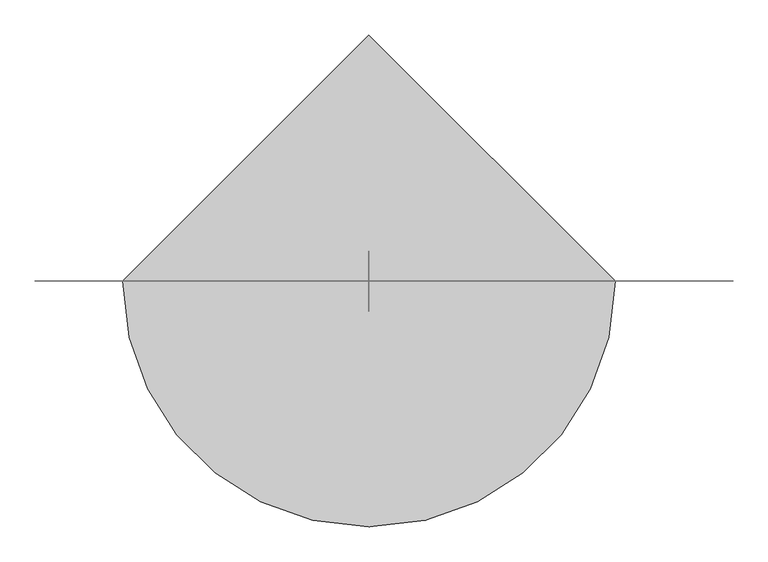
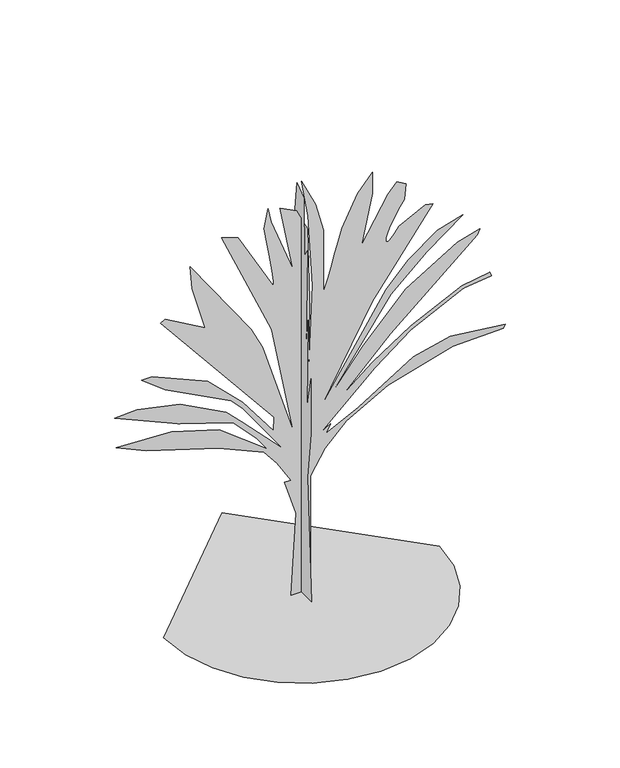
"""IFC4 building model written with IfcOpenShell, lengths in millimetres: proxy geometry, travelers palm 26121 : travelers palm 26121."""

import ifcopenshell
import ifcopenshell.guid

model = None  # the IFC model being written
_history = None  # IfcOwnerHistory: only IFC2X3 demands one
_inside = {}  # id of a spatial element -> (the spatial element, [elements in it])
_under = {}  # id of a project, library or spatial element -> (it, [spatial elements below it])
_declared = {}  # id of a project -> (the project, [libraries it declares])
_typed = {}  # id of a type object -> (the type object, [elements of that type])
_made_of = {}  # id of a material, layer set ... -> (it, [elements and type objects made of it])


def new_model(schema):
    """Start an empty IFC model of exactly this schema.

    Asked for "IFC4X3", IfcOpenShell would pick the latest addendum, in which some entities
    have other attributes; the version numbers below select the first issue.
    IFC2X3 requires an IfcOwnerHistory on every rooted entity: one is made here for all.
    """
    global model, _history
    if schema == "IFC4X3":
        model = ifcopenshell.file(schema_version=(4, 3, 0, 0))
    else:
        model = ifcopenshell.file(schema=schema)
    _inside.clear()
    _under.clear()
    _declared.clear()
    _typed.clear()
    _made_of.clear()
    _history = None
    if model.schema == "IFC2X3":
        org = make("IfcOrganization", Name="unknown")
        user = make(
            "IfcPersonAndOrganization",
            ThePerson=make("IfcPerson", FamilyName="unknown"),
            TheOrganization=org,
        )
        app = make(
            "IfcApplication",
            ApplicationDeveloper=org,
            Version="unknown",
            ApplicationFullName="unknown",
            ApplicationIdentifier="unknown",
        )
        _history = make(
            "IfcOwnerHistory",
            OwningUser=user,
            OwningApplication=app,
            ChangeAction="ADDED",
            CreationDate=0,
        )
    return model


def make(cls, **values):
    """One entity of the class cls with the attributes given. An attribute that is None is left unset."""
    return model.create_entity(
        cls, **{name: value for name, value in values.items() if value is not None}
    )


def rooted(cls, **values):
    """An entity with a GlobalId (a new one), such as an element, a storey or a relation."""
    return make(cls, GlobalId=ifcopenshell.guid.new(), OwnerHistory=_history, **values)


def si_unit(unit_type, name, prefix=None):
    """IfcSIUnit, for example si_unit("LENGTHUNIT", "METRE", prefix="MILLI")."""
    return make("IfcSIUnit", UnitType=unit_type, Prefix=prefix, Name=name)


def assignment(units):
    """IfcUnitAssignment: the units of a project."""
    return None if units is None else make("IfcUnitAssignment", Units=units)


def point(xyz):
    """IfcCartesianPoint."""
    return None if xyz is None else make("IfcCartesianPoint", Coordinates=xyz)


def direction(xyz):
    """IfcDirection."""
    return None if xyz is None else make("IfcDirection", DirectionRatios=xyz)


def frame(location, z_axis=None, x_axis=None):
    """IfcAxis2Placement3D, a coordinate frame: its origin and axes. An axis left out is left unset."""
    return make(
        "IfcAxis2Placement3D",
        Location=point(location),
        Axis=direction(z_axis),
        RefDirection=direction(x_axis),
    )


def origin():
    """The frame at (0, 0, 0) with its axes left unset."""
    return frame((0.0, 0.0, 0.0))


def place(relative_to, where):
    """IfcLocalPlacement: puts the frame where relative to a parent placement (None: the world)."""
    return make(
        "IfcLocalPlacement", PlacementRelTo=relative_to, RelativePlacement=where
    )


def context(
    kind, dimensions, precision=None, world=None, true_north=None, identifier=None
):
    """IfcGeometricRepresentationContext, for example the 3D "Model" context."""
    return make(
        "IfcGeometricRepresentationContext",
        ContextIdentifier=identifier,
        ContextType=kind,
        CoordinateSpaceDimension=dimensions,
        Precision=precision,
        WorldCoordinateSystem=world,
        TrueNorth=true_north,
    )


def project(units=None, contexts=None):
    """IfcProject with its units and contexts."""
    return rooted(
        "IfcProject",
        Name="project",
        RepresentationContexts=contexts,
        UnitsInContext=assignment(units),
    )


def spatial(cls, under=None, at=None, **own):
    """A site, building, storey or space (cls), placed at a placement, below another one or the project."""
    s = rooted(cls, ObjectPlacement=at, **own)
    if under is not None:
        _under.setdefault(under.id(), (under, []))[1].append(s)
    return s


def point_list(points):
    """IfcCartesianPointList2D or 3D."""
    cls = (
        "IfcCartesianPointList2D" if len(points[0]) == 2 else "IfcCartesianPointList3D"
    )
    return make(cls, CoordList=points)


def triangles(points, corners, closed=None, point_numbers=None):
    """IfcTriangulatedFaceSet: each triangle names its three corners, points numbered from 1."""
    return make(
        "IfcTriangulatedFaceSet",
        Coordinates=point_list(points),
        Closed=closed,
        CoordIndex=corners,
        PnIndex=point_numbers,
    )


def shape(context_of_items, identifier, shape_type, items):
    """IfcShapeRepresentation: the items that make up one representation, for example the "Body"."""
    return make(
        "IfcShapeRepresentation",
        ContextOfItems=context_of_items,
        RepresentationIdentifier=identifier,
        RepresentationType=shape_type,
        Items=items,
    )


def source(mapping_origin, context_of_items, identifier, shape_type, items):
    """IfcRepresentationMap: a shape defined once, which mapped items show again and again."""
    return make(
        "IfcRepresentationMap",
        MappingOrigin=mapping_origin,
        MappedRepresentation=shape(context_of_items, identifier, shape_type, items),
    )


def transform(
    local_origin,
    x_axis=None,
    y_axis=None,
    z_axis=None,
    scale=None,
    scale2=None,
    scale3=None,
    uniform=True,
):
    """IfcCartesianTransformationOperator3D, or its non-uniform kind. x_axis, y_axis, z_axis: its Axis1, 2, 3."""
    if uniform:
        return make(
            "IfcCartesianTransformationOperator3D",
            Axis1=direction(x_axis),
            Axis2=direction(y_axis),
            LocalOrigin=point(local_origin),
            Scale=scale,
            Axis3=direction(z_axis),
        )
    return make(
        "IfcCartesianTransformationOperator3DnonUniform",
        Axis1=direction(x_axis),
        Axis2=direction(y_axis),
        LocalOrigin=point(local_origin),
        Scale=scale,
        Axis3=direction(z_axis),
        Scale2=scale2,
        Scale3=scale3,
    )


def mapped(mapping_source, mapping_target):
    """IfcMappedItem: shows the shape of a source again, moved by a transform."""
    return make(
        "IfcMappedItem", MappingSource=mapping_source, MappingTarget=mapping_target
    )


def made_of(thing, what):
    """Note that an element or type object is made of a material, layer set ...; save() writes the relation."""
    if what is not None:
        _made_of.setdefault(what.id(), (what, []))[1].append(thing)
    return thing


def element(
    cls,
    number,
    at=None,
    inside=None,
    cuts=None,
    type_object=None,
    material=None,
    context=None,
    identifier="Body",
    shape_type=None,
    held_by="IfcProductDefinitionShape",
    body=None,
    shapes=None,
    **own,
):
    """One element of the class cls, such as IfcWall. Its Tag is "e" and its number.

    at: its placement. inside: the storey or other place that contains it. cuts: it is an
    opening in that element (IfcRelVoidsElement). A single representation is given by context,
    identifier, shape_type and body (its items); several are given by shapes. held_by: the class
    of the entity that holds the representations. save() writes the other relations.
    """
    e = rooted(cls, Tag="e%d" % number, ObjectPlacement=at, **own)
    if body is not None:
        shapes = [shape(context, identifier, shape_type, body)]
    if shapes is not None:
        e.Representation = make(held_by, Representations=shapes)
    if inside is not None:
        _inside.setdefault(inside.id(), (inside, []))[1].append(e)
    if cuts is not None:
        rooted(
            "IfcRelVoidsElement", RelatingBuildingElement=cuts, RelatedOpeningElement=e
        )
    if type_object is not None:
        _typed.setdefault(type_object.id(), (type_object, []))[1].append(e)
    return made_of(e, material)


def aggregate(whole, parts):
    """IfcRelAggregates: a whole, such as a stair, and the parts it consists of."""
    return rooted("IfcRelAggregates", RelatingObject=whole, RelatedObjects=parts)


def save(model, path):
    """Write the relations noted so far, then the file.

    IfcRelAggregates (storeys below a building ...), IfcRelContainedInSpatialStructure (elements
    in a storey), IfcRelDefinesByType, IfcRelAssociatesMaterial and IfcRelDeclares: one each for
    every whole, place, type object, material and project.
    """
    for whole, parts in _under.values():
        aggregate(whole, parts)
    for where, things in _inside.values():
        rooted(
            "IfcRelContainedInSpatialStructure",
            RelatedElements=things,
            RelatingStructure=where,
        )
    for kind, things in _typed.values():
        rooted("IfcRelDefinesByType", RelatedObjects=things, RelatingType=kind)
    for what, things in _made_of.values():
        rooted("IfcRelAssociatesMaterial", RelatedObjects=things, RelatingMaterial=what)
    for by, libraries in _declared.values():
        rooted("IfcRelDeclares", RelatingContext=by, RelatedDefinitions=libraries)
    model.write(path)


def entourage_0177ab4a(model_context):
    return source(origin(), model_context, "Body", "Tessellation", [
        triangles([(-93.7534889, -0.0079219, 0.0614497), (-47.9158571, -0.0079683, 779.2394274), (-154.8704887, -0.0079884, 1115.3806829), (-93.7534889, -0.0079881, 1110.2879705), (-221.0799467, -0.0080005, 1319.1040764), (-343.3142189, -0.0080096, 1471.8953316), (-755.8511021, -0.0080203, 1650.1526196), (-1417.9506592, -0.0080327, 1858.9686527), (-1692.9744244, -0.0080403, 1986.2938751), (-1183.6685932, -0.0080388, 1960.827697), (-750.7583897, -0.0080309, 1828.4099075), (-312.7554374, -0.0080109, 1492.2660358), (-409.5244217, -0.008019, 1629.7791538), (-623.4331673, -0.0080324, 1853.8733242), (-1122.5511028, -0.0080421, 2016.8526203), (-1708.2550323, -0.0080576, 2276.5982483), (-1499.4389992, -0.0080582, 2286.7861439), (-1107.2729656, -0.008053, 2200.2026207), (-689.6408993, -0.0080397, 1976.1084503), (-547.0350326, -0.0080312, 1833.5026199), (-170.149607, -0.0080081, 1446.4291534), (-531.7569317, -0.0080385, 1955.7349846), (-643.8040169, -0.0080455, 2072.8773983), (-1244.7860836, -0.0080643, 2388.6453335), (-1458.6948292, -0.0080743, 2556.7145805), (-1361.9258812, -0.0080743, 2556.7145805), (-857.7127625, -0.0080609, 2332.6230263), (-536.8496078, -0.0080424, 2021.9453327), (-256.7306412, -0.00802, 1645.0599072), (-251.6384557, -0.0080279, 1777.4776966), (-1285.5302536, -0.0081034, 3045.6393883), (-1244.7860836, -0.008105, 3071.1157402), (-878.0860828, -0.0080922, 2857.1968208), (-1000.3185928, -0.0081174, 3279.9291573), (-1015.5992735, -0.0081302, 3493.8480766), (-460.4539802, -0.0080828, 2699.3102371), (-353.4996074, -0.00807, 2485.4142815), (-73.3816582, -0.0080157, 1573.756992), (-272.0112855, -0.0080789, 2633.1177658), (-730.3875401, -0.0081411, 3677.1854324), (-577.5937778, -0.0081377, 3621.1783859), (-261.8258789, -0.0081041, 3055.8248131), (-253.7766246, -0.0081039, 3053.36101), (-254.8154783, -0.0081061, 3089.6323425), (-263.4286335, -0.0081101, 3158.2124588), (-278.0996675, -0.0081158, 3252.5988487), (-297.3122485, -0.0081226, 3366.3907402), (-319.5550223, -0.0081301, 3493.0862045), (-343.3142189, -0.008138, 3626.2583084), (-302.5700489, -0.0081487, 3804.5157417), (-277.1039979, -0.0081408, 3672.1055099), (-78.4743615, -0.0081092, 3142.4134232), (-195.6149131, -0.0081469, 3773.9594673), (-42.8231537, -0.0081423, 3697.556282), (53.9453128, -0.0081299, 3488.742865), (74.3173933, -0.0080886, 2796.084272), (64.1312281, -0.008043, 2032.1306122), (99.7824359, -0.0080965, 2928.5200836), (59.0382705, -0.0081371, 3610.9929611), (3.0145246, -0.0081581, 3962.4023254), (130.3409359, -0.0081423, 3697.556282), (201.643851, -0.0081259, 3422.5503937), (201.643851, -0.008091, 2836.8259712), (206.54377, -0.0080912, 2840.5597549), (220.2640989, -0.0080935, 2878.5074387), (241.3341791, -0.0080974, 2944.9539642), (268.285114, -0.0081028, 3034.2095627), (299.6439739, -0.0081091, 3140.5594666), (333.9441513, -0.0081161, 3258.339196), (369.7149693, -0.0081235, 3381.7834053), (512.3208361, -0.0081405, 3667.0000076), (649.833954, -0.0081499, 3824.8865913), (649.833954, -0.0081377, 3621.1783859), (547.9722937, -0.0081101, 3157.7043503), (792.4397844, -0.0081341, 3560.0405479), (873.9281244, -0.0081399, 3656.8145828), (955.4164644, -0.0081368, 3605.8877495), (940.1383272, -0.0081283, 3463.2918022), (902.2287952, -0.0081247, 3401.3412231), (866.0592007, -0.008121, 3341.0669952), (833.3617779, -0.0081176, 3284.0693115), (805.8763916, -0.0081145, 3232.0248138), (785.3405085, -0.0081119, 3186.5842735), (773.4913771, -0.0081096, 3149.3731728), (772.066464, -0.008108, 3122.0428642), (778.9574678, -0.0081071, 3107.4885201), (790.3900549, -0.008107, 3106.0406433), (805.6096928, -0.0081076, 3115.4894852), (823.8595963, -0.0081087, 3133.6758751), (844.3802914, -0.0081102, 3158.4156441), (866.4147749, -0.0081119, 3187.5240417), (889.2062616, -0.0081138, 3218.8168991), (1133.6737524, -0.008121, 3341.0417061), (1199.8839552, -0.0081201, 3325.7763588), (649.833954, -0.0080755, 2577.0854301), (171.0856145, -0.0080239, 1711.2701099), (772.066464, -0.0080798, 2648.3834038), (975.7897848, -0.0080925, 2862.3023232), (1240.6281979, -0.0081041, 3055.8248131), (1474.9102638, -0.0081083, 3127.1480759), (1148.9544331, -0.0080937, 2882.6728821), (817.9058899, -0.0080761, 2587.2708549), (247.4814783, -0.0080279, 1777.4776966), (568.3456504, -0.0080521, 2184.9244835), (950.323752, -0.0080764, 2592.3763573), (1423.9781982, -0.0080934, 2877.5676704), (1632.7942314, -0.0080968, 2933.6000061), (1607.3281986, -0.008094, 2887.7783844), (812.810634, -0.0080537, 2210.3880455), (369.7149693, -0.0080272, 1767.2924171), (649.833954, -0.0080406, 1991.3865875), (1001.2558903, -0.0080543, 2220.5759411), (1464.7223682, -0.0080676, 2444.6699661), (1724.470467, -0.00807, 2485.4142815), (1734.6558918, -0.0080676, 2444.6699661), (1480.0029762, -0.0080658, 2414.1113663), (1001.2558903, -0.0080518, 2179.8317711), (670.2048037, -0.008037, 1930.2715679), (181.271766, -0.0080099, 1476.9878986), (267.853309, -0.0080133, 1533.012822), (227.1093933, -0.0080084, 1451.5218658), (522.5062245, -0.0080172, 1599.2204086), (1021.6266672, -0.0080361, 1914.9909599), (1362.8631786, -0.0080406, 1991.3865875), (1861.983585, -0.0080373, 1935.3642803), (1846.702977, -0.0080351, 1899.7128227), (1383.2340282, -0.0080345, 1889.5247818), (792.4397844, -0.0080242, 1716.3628223), (410.4591393, -0.0080118, 1507.5467892), (216.9232418, -0.0080002, 1314.0087479), (84.5035629, -0.0079872, 1095.0072899), (84.5035629, -0.0079219, 0.0), (0.0460873, 53.9902683, 0.0519176), (0.0460761, -156.8964007, 0.0519049), (0.0460873, -97.584823, 1166.5210207), (0.0460761, -150.306614, 1621.2474072), (0.0460761, -150.3063596, 2148.4652264), (0.0460873, -90.9945366, 1832.1335175), (0.0460873, -104.1746006, 2688.8710487), (0.0460873, -71.2236731, 2379.1228043), (0.0460873, -97.584823, 3354.4783859), (0.0460873, -51.4530639, 3275.3826324), (0.0460873, -44.8630274, 3828.9758766), (0.0460982, 67.1710998, 3908.0460503), (0.0460982, 133.0732182, 3374.239389), (0.0460982, 152.8438319, 2609.7752953), (0.0460982, 106.7123182, 1950.7591255), (0.0460873, 53.9902683, 1120.3895342), (-1259.0684967, 0.0, 0.0575648), (-1225.7818657, -288.495908, 0.0575478), (-1130.983873, -553.4307541, 0.0575321), (-982.2667877, -787.2201176, 0.0575181), (-787.2201176, -982.2667877, 0.0575064), (-553.4307541, -1130.983873, 0.0574975), (-288.495908, -1225.7818657, 0.0574919), (4.41e-05, -1259.0684967, 0.0574899), (288.495908, -1225.7818657, 0.0574919), (553.4307541, -1130.983873, 0.0574975), (787.2201176, -982.2667877, 0.0575064), (982.2667877, -787.2201176, 0.0575181), (1130.983873, -553.4307541, 0.0575321), (1225.7818657, -288.495908, 0.0575478), (1259.0684967, 0.0001101, 0.0575648), (-0.0001766, 1259.0684967, 0.05764)], [[59, 60, 61], [99, 100, 101], [8, 9, 10], [49, 50, 51], [98, 99, 101], [15, 16, 17], [15, 17, 18], [119, 120, 121], [34, 35, 36], [33, 34, 36], [98, 101, 102], [97, 98, 102], [24, 25, 26], [24, 26, 27], [23, 24, 27], [23, 27, 28], [22, 23, 28], [22, 28, 29], [21, 22, 29], [7, 8, 10], [7, 10, 11], [71, 72, 73], [106, 107, 108], [106, 108, 109], [105, 106, 109], [104, 105, 109], [104, 109, 110], [103, 104, 110], [39, 40, 41], [39, 41, 42], [52, 53, 54], [52, 54, 55], [52, 55, 56], [59, 61, 62], [58, 59, 62], [58, 62, 63], [57, 58, 63], [7, 11, 12], [6, 7, 12], [15, 18, 19], [14, 15, 19], [14, 19, 20], [13, 14, 20], [13, 20, 21], [12, 13, 21], [93, 94, 95], [92, 93, 95], [91, 92, 95], [90, 91, 95], [89, 90, 95], [88, 89, 95], [87, 88, 95], [2, 3, 4], [96, 97, 102], [96, 102, 103], [124, 125, 126], [124, 126, 127], [39, 42, 43], [49, 51, 52], [48, 49, 52], [47, 48, 52], [46, 47, 52], [45, 46, 52], [44, 45, 52], [86, 87, 95], [114, 115, 116], [113, 114, 116], [30, 31, 32], [30, 32, 33], [30, 33, 36], [30, 36, 37], [30, 37, 38], [29, 30, 38], [21, 29, 38], [131, 132, 1], [131, 1, 2], [131, 2, 4], [5, 6, 12], [5, 12, 21], [123, 124, 127], [123, 127, 128], [122, 123, 128], [122, 128, 129], [121, 122, 129], [121, 129, 130], [113, 116, 117], [112, 113, 117], [111, 112, 117], [111, 117, 118], [110, 111, 118], [110, 118, 119], [103, 110, 119], [96, 103, 119], [71, 73, 74], [70, 71, 74], [69, 70, 74], [68, 69, 74], [44, 52, 56], [43, 44, 56], [39, 43, 56], [39, 56, 57], [38, 39, 57], [75, 76, 77], [75, 77, 78], [74, 75, 78], [74, 78, 79], [74, 79, 80], [74, 80, 81], [74, 81, 82], [74, 82, 83], [74, 83, 84], [74, 84, 85], [67, 68, 74], [119, 121, 130], [130, 131, 4], [130, 4, 5], [130, 5, 21], [119, 130, 21], [119, 21, 38], [96, 119, 38], [96, 38, 57], [95, 96, 57], [95, 57, 63], [95, 63, 64], [86, 95, 64], [86, 64, 65], [86, 65, 66], [86, 66, 67], [86, 67, 74], [86, 74, 85], [138, 139, 140], [136, 137, 138], [140, 141, 142], [143, 144, 145], [142, 143, 145], [142, 145, 146], [140, 142, 146], [140, 146, 147], [138, 140, 147], [138, 147, 148], [136, 138, 148], [135, 136, 148], [134, 135, 148], [134, 148, 133], [163, 164, 149], [162, 163, 149], [162, 149, 150], [161, 162, 150], [161, 150, 151], [161, 151, 152], [160, 161, 152], [159, 160, 152], [159, 152, 153], [159, 153, 154], [159, 154, 155], [159, 155, 156], [159, 156, 157], [159, 157, 158]], closed=False),
    ])


if __name__ == "__main__":
    model = new_model("IFC4")
    model_context = context("Model", 3, world=origin())
    ifc_project = project(units=[si_unit("LENGTHUNIT", "METRE", prefix="MILLI")], contexts=[model_context])
    site = spatial("IfcSite", under=ifc_project)
    building = spatial("IfcBuilding", under=site)
    placement = place(None, origin())
    entourage_shape = entourage_0177ab4a(model_context)
    element("IfcBuildingElementProxy", 1, Name="travelers palm 26121 : travelers palm 26121", ObjectType="travelers palm 26121 : travelers palm 26121", at=placement, inside=building, context=model_context, shape_type="MappedRepresentation", body=[
        mapped(entourage_shape, transform((0.0, 0.0, 0.0), x_axis=(1.0, 0.0, 0.0), y_axis=(0.0, 1.0, 0.0), z_axis=(0.0, 0.0, 1.0))),
    ])
    save(model, "model.ifc")

# Revit data of these elements
# Type "travelers palm 26121 : travelers palm 26121"
#   built-in parameter 1005195 = "RPC-16-G2M6-EAFX-C5H6-W000-ST1L-LVER-AU"
#   Height = 0
